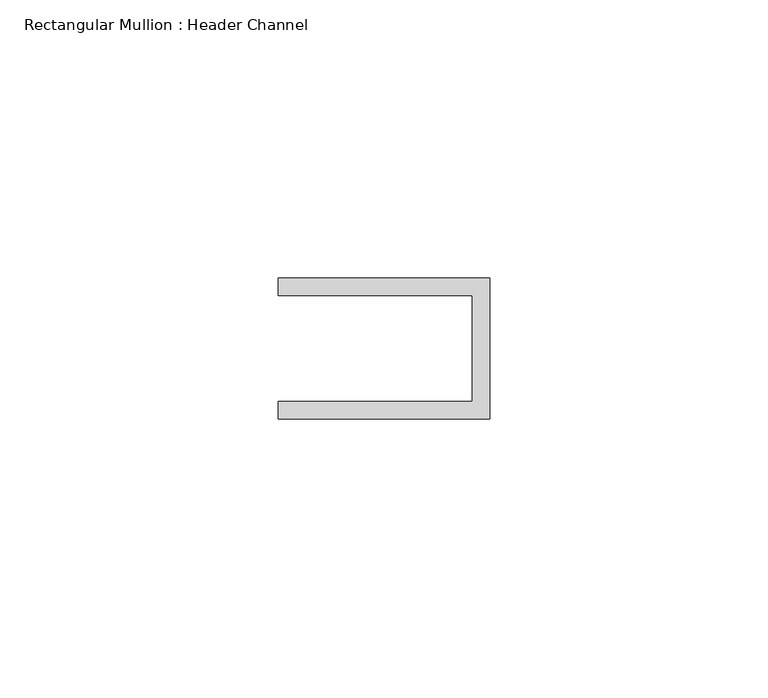
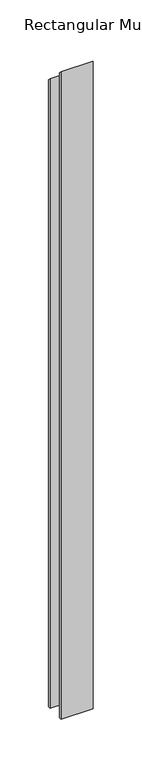
"""IFC4 building model written with IfcOpenShell, lengths in millimetres: member geometry, Rectangular Mullion : Header Channel."""

from ifc_helpers import new_model, si_unit, origin, place, context, project, spatial, faceted_brep, source, transform, mapped, element, save


def rectangular_mullion_header_channel_1d4ec0ec(model_context):
    return source(origin(), model_context, "Body", "Brep", [
        faceted_brep([(0.0, -12.7, -797.4591001), (-38.1, -12.7, -797.4591001), (-38.1, -9.525, -797.4591001), (-3.175, -9.525, -797.4591001), (-3.175, 9.525, -797.4591001), (-38.1, 9.525, -797.4591001), (-38.1, 12.7, -797.4591001), (0.0, 12.7, -797.4591001), (0.0, 12.7, -12.7), (0.0, -12.7, 12.7), (-38.1, 12.7, -12.7), (-38.1, 9.525, -9.525), (-3.175, 9.525, -9.525), (-3.175, -9.525, 9.525), (-38.1, -9.525, 9.525), (-38.1, -12.7, 12.7)], [[[0, 1, 2, 3, 4, 5, 6, 7]], [[8, 9, 0, 7]], [[10, 8, 7, 6]], [[11, 10, 6, 5]], [[12, 11, 5, 4]], [[13, 12, 4, 3]], [[14, 13, 3, 2]], [[15, 14, 2, 1]], [[9, 15, 1, 0]], [[9, 8, 10, 11, 12, 13, 14, 15]]]),
    ])


if __name__ == "__main__":
    model = new_model("IFC4")
    model_context = context("Model", 3, world=origin())
    ifc_project = project(units=[si_unit("LENGTHUNIT", "METRE", prefix="MILLI")], contexts=[model_context])
    site = spatial("IfcSite", under=ifc_project)
    building = spatial("IfcBuilding", under=site)
    placement = place(None, origin())
    rectangular_mullion_header_channel_shape = rectangular_mullion_header_channel_1d4ec0ec(model_context)
    element("IfcMember", 1, ObjectType="Rectangular Mullion : Header Channel", at=placement, inside=building, context=model_context, shape_type="MappedRepresentation", body=[
        mapped(rectangular_mullion_header_channel_shape, transform((0.0, 0.0, 0.0), x_axis=(1.0, 0.0, 0.0), y_axis=(0.0, 1.0, 0.0), z_axis=(0.0, 0.0, 1.0))),
    ])
    save(model, "model.ifc")

# Revit data of these elements
# Type "Rectangular Mullion : Header Channel"
#   built-in parameter 1007322 = 0.0833333 (stored number, unit not read)
#   built-in parameter 1007321 = -0.03125 (stored number, unit not read)
#   built-in parameter 1007320 = 0.0416667 (stored number, unit not read)
# Element 1 (IfcMember, "Rectangular Mullion : Header Channel")
#   Materials on its faces: "ALUM"
# Materials
#   "ALUM": class "Generic", colour RGB 157 157 157, transparency 0, Cost = 0
